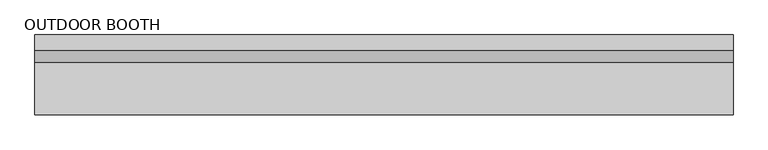
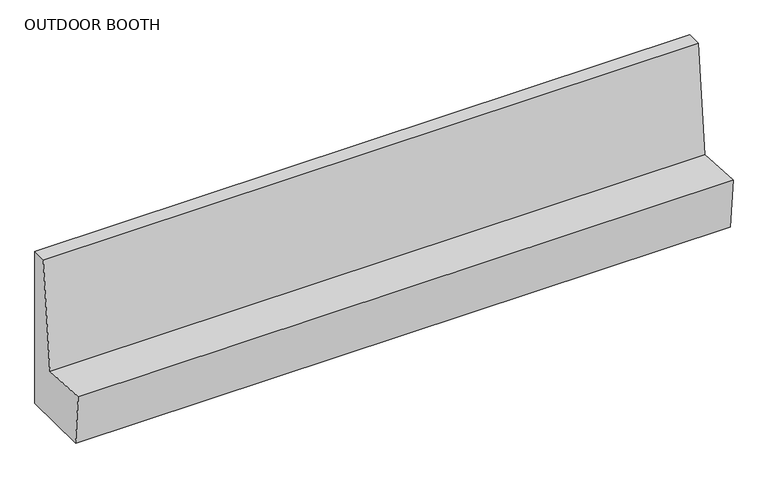
"""IFC4 building model written with IfcOpenShell, lengths in millimetres: furniture geometry, OD_CW_Booth : OUTDOOR BOOTH."""

from ifc_helpers import new_model, si_unit, frame, origin, place, context, project, spatial, polyline, outline, extrude, source, transform, mapped, element, save


def outdoor_booth_dbb49056(model_context):
    return source(origin(), model_context, "Body", "SweptSolid", [
        extrude(outline(polyline([(609.6, 1397.0), (609.6, 0.0), (-3.4100193, 0.0), (-43.0849153, 453.4861359), (382.9385128, 431.1591941), (484.4524721, 1397.0), (609.6, 1397.0)])), frame((18.7377049, 0.0, 0.0), z_axis=(1.0, 0.0, 0.0), x_axis=(0.0, 1.0, 0.0)), (0.0, 0.0, 1.0), 5700.9355441),
    ])


if __name__ == "__main__":
    model = new_model("IFC4")
    model_context = context("Model", 3, world=origin())
    ifc_project = project(units=[si_unit("LENGTHUNIT", "METRE", prefix="MILLI")], contexts=[model_context])
    site = spatial("IfcSite", under=ifc_project)
    building = spatial("IfcBuilding", under=site)
    placement = place(None, origin())
    outdoor_booth_shape = outdoor_booth_dbb49056(model_context)
    element("IfcFurniture", 1, ObjectType="OD_CW_Booth : OUTDOOR BOOTH", at=placement, inside=building, context=model_context, shape_type="MappedRepresentation", body=[
        mapped(outdoor_booth_shape, transform((0.0, 0.0, 0.0), x_axis=(1.0, 0.0, 0.0), y_axis=(0.0, 1.0, 0.0), z_axis=(0.0, 0.0, 1.0))),
    ])
    save(model, "model.ifc")

# Revit data of these elements
# Type "OD_CW_Booth : OUTDOOR BOOTH"
#   Type Mark = "TYPE-OUTDOOR"
#   Width = 4' - 0"
#   OD_CW_Width [instance default] = 2' - 10"
#   OD_CW_Length [instance default] = 26' - 1 83/256"
#   OD_CW_Height [instance default] = 2' - 3"
#   Height = 3' - 0"
#   Depth = 2' - 0"
#   Seating Count [instance default] = 10
#   OD_CW_Material_Front Panel [instance default] = none
#   OD_CW_Material_Body [instance default] = none
# Element 1 (IfcFurniture, "OD_CW_Booth : OUTDOOR BOOTH")
#   OD_CW_Length = 18' - 8.44628"
#   Seating Count = 7
#   OD_CW_Material_Body = Sals Wood
#   Materials on its faces: "Sals Wood"
# Materials
#   "Sals Wood": class "Wood", colour RGB 198 202 183, transparency 0, Description = "Generic wood", Cost = 0
